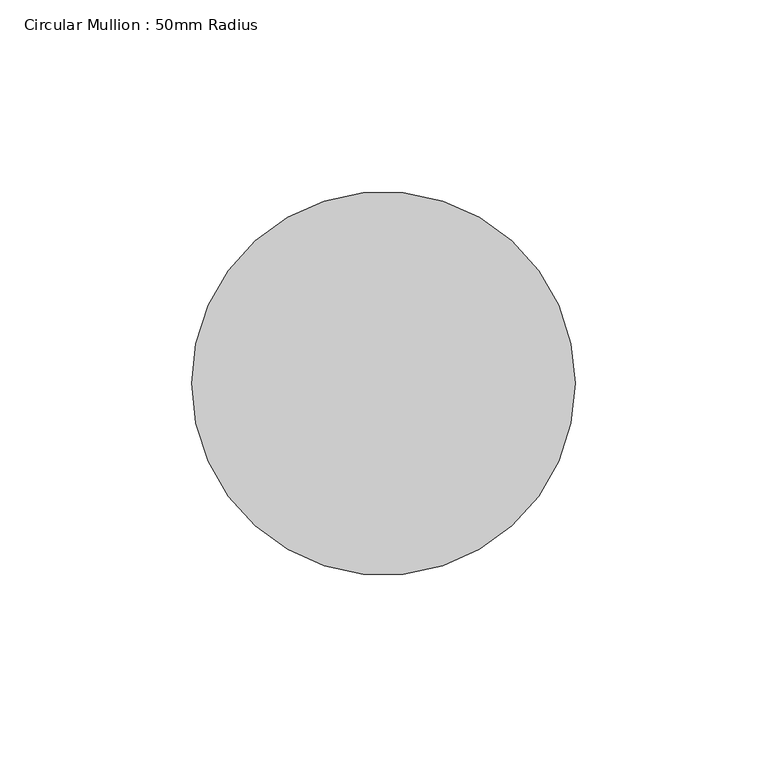
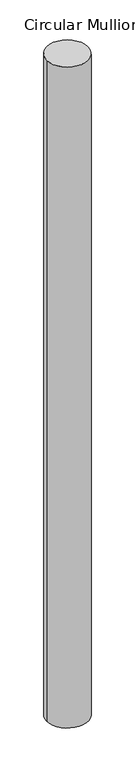
"""IFC4 building model written with IfcOpenShell, lengths in millimetres: member geometry, Circular Mullion : 50mm Radius."""

from ifc_helpers import new_model, si_unit, point, frame, origin, origin_2d, place, context, project, spatial, circle_curve, trimmed, segment, composite_curve, outline, extrude, source, transform, mapped, element, save


def circular_mullion_50mm_radius_62509d0d(model_context):
    return source(origin(), model_context, "Body", "SweptSolid", [
        extrude(outline(composite_curve([segment(trimmed(circle_curve(origin_2d(), 50.0), [point((50.0, 0.0))], [point((-50.0, 0.0))], False, "CARTESIAN"), True, "CONTINUOUS"), segment(trimmed(circle_curve(origin_2d(), 50.0), [point((-50.0, 0.0))], [point((50.0, 0.0))], False, "CARTESIAN"), True, "CONTINUOUS")], self_intersect=False)), frame((0.0, 0.0, -1699.7284385), z_axis=(0.0, 0.0, 1.0), x_axis=(1.0, 0.0, 0.0)), (0.0, 0.0, 1.0), 1699.7284385),
    ])


if __name__ == "__main__":
    model = new_model("IFC4")
    model_context = context("Model", 3, world=origin())
    ifc_project = project(units=[si_unit("LENGTHUNIT", "METRE", prefix="MILLI")], contexts=[model_context])
    site = spatial("IfcSite", under=ifc_project)
    building = spatial("IfcBuilding", under=site)
    placement = place(None, origin())
    circular_mullion_50mm_radius_shape = circular_mullion_50mm_radius_62509d0d(model_context)
    element("IfcMember", 1, ObjectType="Circular Mullion : 50mm Radius", at=placement, inside=building, context=model_context, shape_type="MappedRepresentation", body=[
        mapped(circular_mullion_50mm_radius_shape, transform((0.0, 0.0, 0.0), x_axis=(1.0, 0.0, 0.0), y_axis=(0.0, 1.0, 0.0), z_axis=(0.0, 0.0, 1.0))),
    ])
    save(model, "model.ifc")

# Revit data of these elements
# Type "Circular Mullion : 50mm Radius"
#   built-in parameter 1007350 = 0.164042 (stored number, unit not read)
# Element 1 (IfcMember, "Circular Mullion : 50mm Radius")
#   Materials on its faces: "Aluminium"
# Materials
#   "Aluminium": class "Metal", colour RGB 247 247 247, transparency 0, Description = "Aluminium 6061", Cost = 0
